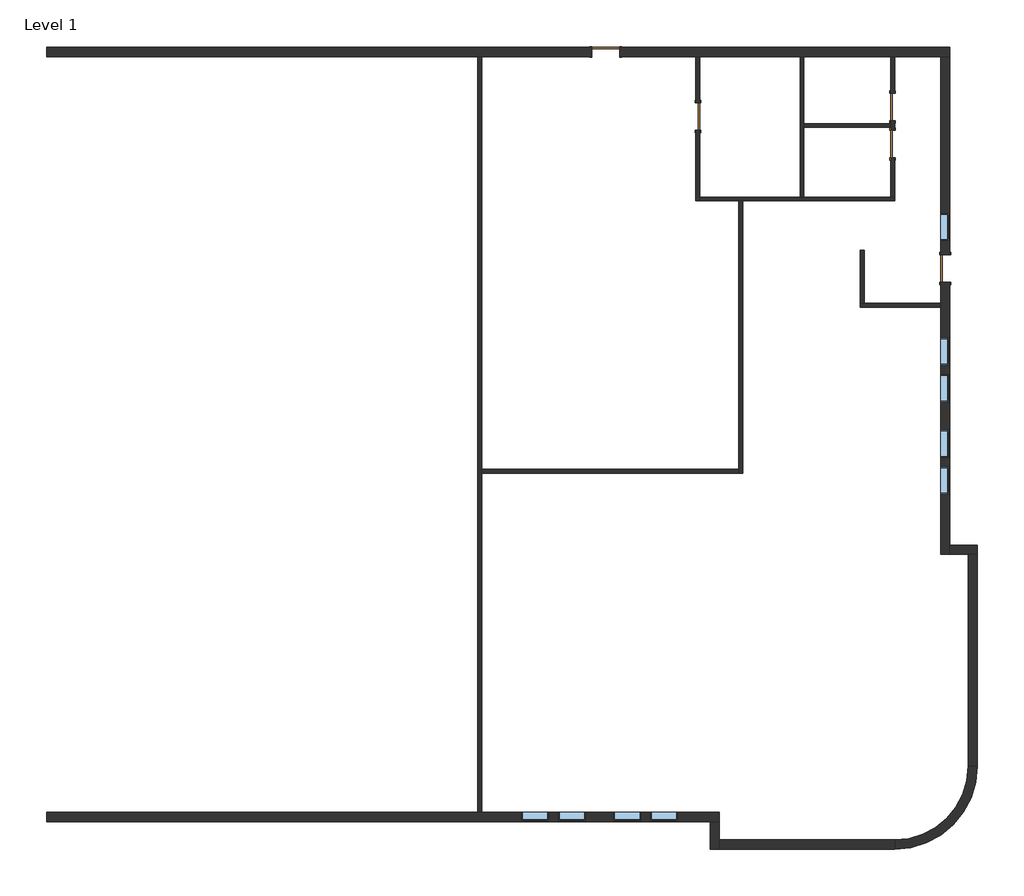
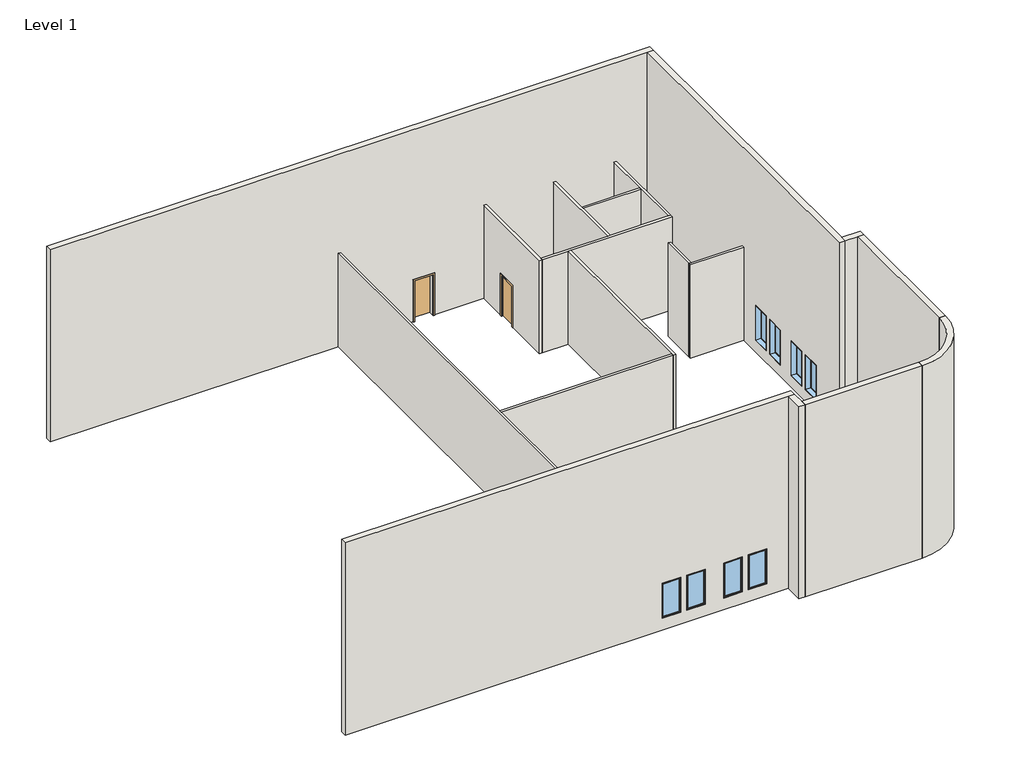
# One storey: 18 walls, 9 windows, 5 doors.
"""IFC4 building model written with IfcOpenShell, lengths in millimetres."""

import ifcopenshell
import ifcopenshell.guid

model = None  # the IFC model being written
_history = None  # IfcOwnerHistory: only IFC2X3 demands one
_inside = {}  # id of a spatial element -> (the spatial element, [elements in it])
_under = {}  # id of a project, library or spatial element -> (it, [spatial elements below it])
_declared = {}  # id of a project -> (the project, [libraries it declares])
_typed = {}  # id of a type object -> (the type object, [elements of that type])
_made_of = {}  # id of a material, layer set ... -> (it, [elements and type objects made of it])


def new_model(schema):
    """Start an empty IFC model of exactly this schema.

    Asked for "IFC4X3", IfcOpenShell would pick the latest addendum, in which some entities
    have other attributes; the version numbers below select the first issue.
    IFC2X3 requires an IfcOwnerHistory on every rooted entity: one is made here for all.
    """
    global model, _history
    if schema == "IFC4X3":
        model = ifcopenshell.file(schema_version=(4, 3, 0, 0))
    else:
        model = ifcopenshell.file(schema=schema)
    _inside.clear()
    _under.clear()
    _declared.clear()
    _typed.clear()
    _made_of.clear()
    _history = None
    if model.schema == "IFC2X3":
        org = make("IfcOrganization", Name="unknown")
        user = make(
            "IfcPersonAndOrganization",
            ThePerson=make("IfcPerson", FamilyName="unknown"),
            TheOrganization=org,
        )
        app = make(
            "IfcApplication",
            ApplicationDeveloper=org,
            Version="unknown",
            ApplicationFullName="unknown",
            ApplicationIdentifier="unknown",
        )
        _history = make(
            "IfcOwnerHistory",
            OwningUser=user,
            OwningApplication=app,
            ChangeAction="ADDED",
            CreationDate=0,
        )
    return model


def make(cls, **values):
    """One entity of the class cls with the attributes given. An attribute that is None is left unset."""
    return model.create_entity(
        cls, **{name: value for name, value in values.items() if value is not None}
    )


def rooted(cls, **values):
    """An entity with a GlobalId (a new one), such as an element, a storey or a relation."""
    return make(cls, GlobalId=ifcopenshell.guid.new(), OwnerHistory=_history, **values)


def si_unit(unit_type, name, prefix=None):
    """IfcSIUnit, for example si_unit("LENGTHUNIT", "METRE", prefix="MILLI")."""
    return make("IfcSIUnit", UnitType=unit_type, Prefix=prefix, Name=name)


def assignment(units):
    """IfcUnitAssignment: the units of a project."""
    return None if units is None else make("IfcUnitAssignment", Units=units)


def point(xyz):
    """IfcCartesianPoint."""
    return None if xyz is None else make("IfcCartesianPoint", Coordinates=xyz)


def direction(xyz):
    """IfcDirection."""
    return None if xyz is None else make("IfcDirection", DirectionRatios=xyz)


def frame(location, z_axis=None, x_axis=None):
    """IfcAxis2Placement3D, a coordinate frame: its origin and axes. An axis left out is left unset."""
    return make(
        "IfcAxis2Placement3D",
        Location=point(location),
        Axis=direction(z_axis),
        RefDirection=direction(x_axis),
    )


def frame_2d(location, x_axis=None):
    """IfcAxis2Placement2D, a coordinate frame in the plane: its origin and x axis."""
    return make(
        "IfcAxis2Placement2D", Location=point(location), RefDirection=direction(x_axis)
    )


def origin():
    """The frame at (0, 0, 0) with its axes left unset."""
    return frame((0.0, 0.0, 0.0))


def origin_with_axes():
    """The frame at (0, 0, 0) with the z axis (0, 0, 1) and the x axis (1, 0, 0) written out."""
    return frame((0.0, 0.0, 0.0), z_axis=(0.0, 0.0, 1.0), x_axis=(1.0, 0.0, 0.0))


def place(relative_to, where):
    """IfcLocalPlacement: puts the frame where relative to a parent placement (None: the world)."""
    return make(
        "IfcLocalPlacement", PlacementRelTo=relative_to, RelativePlacement=where
    )


def context(
    kind, dimensions, precision=None, world=None, true_north=None, identifier=None
):
    """IfcGeometricRepresentationContext, for example the 3D "Model" context."""
    return make(
        "IfcGeometricRepresentationContext",
        ContextIdentifier=identifier,
        ContextType=kind,
        CoordinateSpaceDimension=dimensions,
        Precision=precision,
        WorldCoordinateSystem=world,
        TrueNorth=true_north,
    )


def project(units=None, contexts=None):
    """IfcProject with its units and contexts."""
    return rooted(
        "IfcProject",
        Name="project",
        RepresentationContexts=contexts,
        UnitsInContext=assignment(units),
    )


def spatial(cls, under=None, at=None, **own):
    """A site, building, storey or space (cls), placed at a placement, below another one or the project."""
    s = rooted(cls, ObjectPlacement=at, **own)
    if under is not None:
        _under.setdefault(under.id(), (under, []))[1].append(s)
    return s


def polyline(points):
    """IfcPolyline through the points."""
    return make("IfcPolyline", Points=[point(p) for p in points])


def circle_curve(where, radius):
    """IfcCircle in the frame where."""
    return make("IfcCircle", Position=where, Radius=radius)


def trimmed(basis, trim1, trim2, sense, master):
    """IfcTrimmedCurve: the piece of a basis curve between two trims."""
    return make(
        "IfcTrimmedCurve",
        BasisCurve=basis,
        Trim1=trim1,
        Trim2=trim2,
        SenseAgreement=sense,
        MasterRepresentation=master,
    )


def segment(curve, same_sense, transition):
    """IfcCompositeCurveSegment."""
    return make(
        "IfcCompositeCurveSegment",
        Transition=transition,
        SameSense=same_sense,
        ParentCurve=curve,
    )


def composite_curve(segments, self_intersect=None):
    """IfcCompositeCurve: segments joined end to end."""
    return make("IfcCompositeCurve", Segments=segments, SelfIntersect=self_intersect)


def outline(outer, holes=None, kind="AREA"):
    """IfcArbitraryClosedProfileDef: a profile drawn as a closed curve; with holes, ...WithVoids."""
    if holes is None:
        return make("IfcArbitraryClosedProfileDef", ProfileType=kind, OuterCurve=outer)
    return make(
        "IfcArbitraryProfileDefWithVoids",
        ProfileType=kind,
        OuterCurve=outer,
        InnerCurves=holes,
    )


def extrude(swept, where, along, depth):
    """IfcExtrudedAreaSolid: the profile swept, set in the frame where, extruded along a direction by depth."""
    return make(
        "IfcExtrudedAreaSolid",
        SweptArea=swept,
        Position=where,
        ExtrudedDirection=direction(along),
        Depth=depth,
    )


def faces_of(points, faces, orient=None, outer=None):
    """IfcFace entities. A face is a list of loops; a loop is a list of indices into points, from 0.

    orient and outer hold one flag for each loop. By default every Orientation is true, the
    first loop of a face is its IfcFaceOuterBound and the others are IfcFaceBound.
    """
    made = []
    for i, loops in enumerate(faces):
        bounds = []
        for j, loop in enumerate(loops):
            is_outer = j == 0 if outer is None else outer[i][j]
            bounds.append(
                make(
                    "IfcFaceOuterBound" if is_outer else "IfcFaceBound",
                    Bound=make("IfcPolyLoop", Polygon=[points[k] for k in loop]),
                    Orientation=True if orient is None else orient[i][j],
                )
            )
        made.append(make("IfcFace", Bounds=bounds))
    return made


def faceted_brep(points, faces, orient=None, outer=None, voids=None):
    """IfcFacetedBrep: a solid bounded by flat faces; with voids (closed shells), ...WithVoids."""
    shared = [point(p) for p in points]
    hull = make("IfcClosedShell", CfsFaces=faces_of(shared, faces, orient, outer))
    if voids is None:
        return make("IfcFacetedBrep", Outer=hull)
    return make(
        "IfcFacetedBrepWithVoids",
        Outer=hull,
        Voids=[
            make(cls, CfsFaces=faces_of(shared, fs, o, b)) for cls, fs, o, b in voids
        ],
    )


def shape(context_of_items, identifier, shape_type, items):
    """IfcShapeRepresentation: the items that make up one representation, for example the "Body"."""
    return make(
        "IfcShapeRepresentation",
        ContextOfItems=context_of_items,
        RepresentationIdentifier=identifier,
        RepresentationType=shape_type,
        Items=items,
    )


def source(mapping_origin, context_of_items, identifier, shape_type, items):
    """IfcRepresentationMap: a shape defined once, which mapped items show again and again."""
    return make(
        "IfcRepresentationMap",
        MappingOrigin=mapping_origin,
        MappedRepresentation=shape(context_of_items, identifier, shape_type, items),
    )


def transform(
    local_origin,
    x_axis=None,
    y_axis=None,
    z_axis=None,
    scale=None,
    scale2=None,
    scale3=None,
    uniform=True,
):
    """IfcCartesianTransformationOperator3D, or its non-uniform kind. x_axis, y_axis, z_axis: its Axis1, 2, 3."""
    if uniform:
        return make(
            "IfcCartesianTransformationOperator3D",
            Axis1=direction(x_axis),
            Axis2=direction(y_axis),
            LocalOrigin=point(local_origin),
            Scale=scale,
            Axis3=direction(z_axis),
        )
    return make(
        "IfcCartesianTransformationOperator3DnonUniform",
        Axis1=direction(x_axis),
        Axis2=direction(y_axis),
        LocalOrigin=point(local_origin),
        Scale=scale,
        Axis3=direction(z_axis),
        Scale2=scale2,
        Scale3=scale3,
    )


def mapped(mapping_source, mapping_target):
    """IfcMappedItem: shows the shape of a source again, moved by a transform."""
    return make(
        "IfcMappedItem", MappingSource=mapping_source, MappingTarget=mapping_target
    )


def made_of(thing, what):
    """Note that an element or type object is made of a material, layer set ...; save() writes the relation."""
    if what is not None:
        _made_of.setdefault(what.id(), (what, []))[1].append(thing)
    return thing


def element(
    cls,
    number,
    at=None,
    inside=None,
    cuts=None,
    type_object=None,
    material=None,
    context=None,
    identifier="Body",
    shape_type=None,
    held_by="IfcProductDefinitionShape",
    body=None,
    shapes=None,
    **own,
):
    """One element of the class cls, such as IfcWall. Its Tag is "e" and its number.

    at: its placement. inside: the storey or other place that contains it. cuts: it is an
    opening in that element (IfcRelVoidsElement). A single representation is given by context,
    identifier, shape_type and body (its items); several are given by shapes. held_by: the class
    of the entity that holds the representations. save() writes the other relations.
    """
    e = rooted(cls, Tag="e%d" % number, ObjectPlacement=at, **own)
    if body is not None:
        shapes = [shape(context, identifier, shape_type, body)]
    if shapes is not None:
        e.Representation = make(held_by, Representations=shapes)
    if inside is not None:
        _inside.setdefault(inside.id(), (inside, []))[1].append(e)
    if cuts is not None:
        rooted(
            "IfcRelVoidsElement", RelatingBuildingElement=cuts, RelatedOpeningElement=e
        )
    if type_object is not None:
        _typed.setdefault(type_object.id(), (type_object, []))[1].append(e)
    return made_of(e, material)


def aggregate(whole, parts):
    """IfcRelAggregates: a whole, such as a stair, and the parts it consists of."""
    return rooted("IfcRelAggregates", RelatingObject=whole, RelatedObjects=parts)


def save(model, path):
    """Write the relations noted so far, then the file.

    IfcRelAggregates (storeys below a building ...), IfcRelContainedInSpatialStructure (elements
    in a storey), IfcRelDefinesByType, IfcRelAssociatesMaterial and IfcRelDeclares: one each for
    every whole, place, type object, material and project.
    """
    for whole, parts in _under.values():
        aggregate(whole, parts)
    for where, things in _inside.values():
        rooted(
            "IfcRelContainedInSpatialStructure",
            RelatedElements=things,
            RelatingStructure=where,
        )
    for kind, things in _typed.values():
        rooted("IfcRelDefinesByType", RelatedObjects=things, RelatingType=kind)
    for what, things in _made_of.values():
        rooted("IfcRelAssociatesMaterial", RelatedObjects=things, RelatingMaterial=what)
    for by, libraries in _declared.values():
        rooted("IfcRelDeclares", RelatingContext=by, RelatedDefinitions=libraries)
    model.write(path)


def door_2bf94977(model_context):
    return source(origin(), model_context, "Body", "SweptSolid", [
        extrude(outline(polyline([(2209.8, -533.4), (0.0, -533.4), (0.0, -457.2), (2133.6, -457.2), (2133.6, 457.2), (0.0, 457.2), (0.0, 533.4), (2209.8, 533.4), (2209.8, -533.4)])), frame((0.0, -177.8, 0.0), z_axis=(0.0, 1.0, 0.0), x_axis=(0.0, 0.0, 1.0)), (0.0, 0.0, 1.0), 25.4),
        extrude(outline(polyline([(2209.8, 533.4), (2209.8, -533.4), (0.0, -533.4), (0.0, -457.2), (2133.6, -457.2), (2133.6, 457.2), (0.0, 457.2), (0.0, 533.4), (2209.8, 533.4)])), frame((0.0, 152.4, 0.0), z_axis=(0.0, 1.0, 0.0), x_axis=(0.0, 0.0, 1.0)), (0.0, 0.0, 1.0), 25.4),
        extrude(outline(polyline([(457.2, -101.6), (457.2, -152.4), (-457.2, -152.4), (-457.2, -101.6), (457.2, -101.6)])), origin_with_axes(), (0.0, 0.0, 1.0), 2133.6),
    ])


def door_a3eb833a(model_context):
    return source(origin(), model_context, "Body", "SweptSolid", [
        extrude(outline(polyline([(2209.8, -533.4), (0.0, -533.4), (0.0, -457.2), (2133.6, -457.2), (2133.6, 457.2), (0.0, 457.2), (0.0, 533.4), (2209.8, 533.4), (2209.8, -533.4)])), frame((0.0, -88.9, 0.0), z_axis=(0.0, 1.0, 0.0), x_axis=(0.0, 0.0, 1.0)), (0.0, 0.0, 1.0), 25.4),
        extrude(outline(polyline([(2209.8, 533.4), (2209.8, -533.4), (0.0, -533.4), (0.0, -457.2), (2133.6, -457.2), (2133.6, 457.2), (0.0, 457.2), (0.0, 533.4), (2209.8, 533.4)])), frame((0.0, 63.5, 0.0), z_axis=(0.0, 1.0, 0.0), x_axis=(0.0, 0.0, 1.0)), (0.0, 0.0, 1.0), 25.4),
        extrude(outline(polyline([(457.2, -12.7), (457.2, -63.5), (-457.2, -63.5), (-457.2, -12.7), (457.2, -12.7)])), origin_with_axes(), (0.0, 0.0, 1.0), 2133.6),
    ])


def door_a1797ceb(model_context):
    return source(origin(), model_context, "Body", "SweptSolid", [
        extrude(outline(polyline([(2209.8, -533.4), (0.0, -533.4), (0.0, -457.2), (2133.6, -457.2), (2133.6, 457.2), (0.0, 457.2), (0.0, 533.4), (2209.8, 533.4), (2209.8, -533.4)])), frame((0.0, 63.5, 0.0), z_axis=(0.0, 1.0, 0.0), x_axis=(0.0, 0.0, 1.0)), (0.0, 0.0, 1.0), 25.4),
        extrude(outline(polyline([(2209.8, 533.4), (2209.8, -533.4), (0.0, -533.4), (0.0, -457.2), (2133.6, -457.2), (2133.6, 457.2), (0.0, 457.2), (0.0, 533.4), (2209.8, 533.4)])), frame((0.0, -88.9, 0.0), z_axis=(0.0, 1.0, 0.0), x_axis=(0.0, 0.0, 1.0)), (0.0, 0.0, 1.0), 25.4),
        extrude(outline(polyline([(457.2, 12.7), (-457.2, 12.7), (-457.2, 63.5), (457.2, 63.5), (457.2, 12.7)])), origin_with_axes(), (0.0, 0.0, 1.0), 2133.6),
    ])


def window_c524ad49(model_context):
    return source(origin(), model_context, "Body", "SweptSolid", [
        extrude(outline(polyline([(355.6, 104.775), (-431.8, 104.775), (-431.8, 117.475), (355.6, 117.475), (355.6, 104.775)])), frame((0.0, 0.0, 368.3), z_axis=(0.0, 0.0, 1.0), x_axis=(1.0, 0.0, 0.0)), (0.0, 0.0, 1.0), 1701.8),
        extrude(outline(polyline([(2114.55, -476.25), (323.85, -476.25), (323.85, 400.05), (2114.55, 400.05), (2114.55, -476.25)]), holes=[polyline([(2070.1, -431.8), (2070.1, 355.6), (368.3, 355.6), (368.3, -431.8), (2070.1, -431.8)])]), frame((0.0, 88.9, 0.0), z_axis=(0.0, 1.0, 0.0), x_axis=(0.0, 0.0, 1.0)), (0.0, 0.0, 1.0), 44.45),
        extrude(outline(polyline([(2133.6, -495.3), (304.8, -495.3), (304.8, 419.1), (2133.6, 419.1), (2133.6, -495.3)]), holes=[polyline([(2101.85, -463.55), (2101.85, 387.35), (336.55, 387.35), (336.55, -463.55), (2101.85, -463.55)])]), frame((0.0, -152.4, 0.0), z_axis=(0.0, 1.0, 0.0), x_axis=(0.0, 0.0, 1.0)), (0.0, 0.0, 1.0), 241.3),
        extrude(outline(polyline([(2133.6, 419.1), (2133.6, -495.3), (304.8, -495.3), (304.8, 419.1), (2133.6, 419.1)]), holes=[polyline([(2114.55, 400.05), (323.85, 400.05), (323.85, -476.25), (2114.55, -476.25), (2114.55, 400.05)])]), frame((0.0, 88.9, 0.0), z_axis=(0.0, 1.0, 0.0), x_axis=(0.0, 0.0, 1.0)), (0.0, 0.0, 1.0), 63.5),
    ])


def window_9a1f8bc2(model_context):
    return source(origin(), model_context, "Body", "SweptSolid", [
        extrude(outline(polyline([(355.6, -104.775), (355.6, -117.475), (-431.8, -117.475), (-431.8, -104.775), (355.6, -104.775)])), frame((0.0, 0.0, 368.3), z_axis=(0.0, 0.0, 1.0), x_axis=(1.0, 0.0, 0.0)), (0.0, 0.0, 1.0), 1701.8),
        extrude(outline(polyline([(2114.55, -476.25), (323.85, -476.25), (323.85, 400.05), (2114.55, 400.05), (2114.55, -476.25)]), holes=[polyline([(2070.1, -431.8), (2070.1, 355.6), (368.3, 355.6), (368.3, -431.8), (2070.1, -431.8)])]), frame((0.0, -133.35, 0.0), z_axis=(0.0, 1.0, 0.0), x_axis=(0.0, 0.0, 1.0)), (0.0, 0.0, 1.0), 44.45),
        extrude(outline(polyline([(2133.6, -495.3), (304.8, -495.3), (304.8, 419.1), (2133.6, 419.1), (2133.6, -495.3)]), holes=[polyline([(2101.85, -463.55), (2101.85, 387.35), (336.55, 387.35), (336.55, -463.55), (2101.85, -463.55)])]), frame((0.0, -88.9, 0.0), z_axis=(0.0, 1.0, 0.0), x_axis=(0.0, 0.0, 1.0)), (0.0, 0.0, 1.0), 241.3),
        extrude(outline(polyline([(2133.6, 419.1), (2133.6, -495.3), (304.8, -495.3), (304.8, 419.1), (2133.6, 419.1)]), holes=[polyline([(2114.55, 400.05), (323.85, 400.05), (323.85, -476.25), (2114.55, -476.25), (2114.55, 400.05)])]), frame((0.0, -152.4, 0.0), z_axis=(0.0, 1.0, 0.0), x_axis=(0.0, 0.0, 1.0)), (0.0, 0.0, 1.0), 63.5),
    ])


model = new_model("IFC4")

# Units and contexts
model_context = context("Model", 3, world=origin())
ifc_project = project(units=[si_unit("LENGTHUNIT", "METRE", prefix="MILLI")], contexts=[model_context])

# Site, building, storey
site = spatial("IfcSite", under=ifc_project)
building = spatial("IfcBuilding", under=site)
storey = spatial("IfcBuildingStorey", under=building, Name="Level 1", Elevation=0.0)

# Doors
placement = place(None, origin())
door_shape = door_2bf94977(model_context)
element("IfcDoor", 1, ObjectType="Single-Flush : 36\" x 84\"", at=placement, inside=storey, context=model_context, shape_type="MappedRepresentation", body=[
    mapped(door_shape, transform((7004.4737178, 13634.9120281, 0.0), x_axis=(-1.0, 0.0, 0.0), y_axis=(0.0, -1.0, 0.0), z_axis=(0.0, 0.0, 1.0))),
])
element("IfcDoor", 2, ObjectType="Single-Flush : 36\" x 84\"", at=placement, inside=storey, context=model_context, shape_type="MappedRepresentation", body=[
    mapped(door_shape, transform((18231.2737178, 6472.1120281, 0.0), x_axis=(0.0, -1.0, 0.0), y_axis=(1.0, 0.0, 0.0), z_axis=(0.0, 0.0, 1.0))),
])
door_2_shape = door_a3eb833a(model_context)
element("IfcDoor", 3, ObjectType="Single-Flush : 36\" x 84\"", at=placement, inside=storey, context=model_context, shape_type="MappedRepresentation", body=[
    mapped(door_2_shape, transform((16491.3737178, 11812.4620281, 0.0), x_axis=(0.0, -1.0, 0.0), y_axis=(1.0, 0.0, 0.0), z_axis=(0.0, 0.0, 1.0))),
])
element("IfcDoor", 4, ObjectType="Single-Flush : 36\" x 84\"", at=placement, inside=storey, context=model_context, shape_type="MappedRepresentation", body=[
    mapped(door_2_shape, transform((10052.4737178, 11501.3120281, 0.0), x_axis=(0.0, 1.0, 0.0), y_axis=(-1.0, 0.0, 0.0), z_axis=(0.0, 0.0, 1.0))),
])
door_3_shape = door_a1797ceb(model_context)
element("IfcDoor", 5, ObjectType="Single-Flush : 36\" x 84\"", at=placement, inside=storey, context=model_context, shape_type="MappedRepresentation", body=[
    mapped(door_3_shape, transform((16491.3737178, 10593.2620281, 0.0), x_axis=(0.0, 1.0, 0.0), y_axis=(-1.0, 0.0, 0.0), z_axis=(0.0, 0.0, 1.0))),
])

# Walls
element("IfcWall", 6, ObjectType="Generic - 12\"", at=placement, inside=storey, context=model_context, shape_type="Brep", body=[
    faceted_brep([(-11486.7262822, 13482.5120281, 0.0), (2775.3737178, 13482.5120281, 0.0), (2902.3737178, 13482.5120281, 0.0), (6547.2737178, 13482.5120281, 0.0), (6547.2737178, 13482.5120281, 2133.6), (7461.6737178, 13482.5120281, 2133.6), (7461.6737178, 13482.5120281, 0.0), (9988.9737178, 13482.5120281, 0.0), (10115.9737178, 13482.5120281, 0.0), (13430.6737178, 13482.5120281, 0.0), (13557.6737178, 13482.5120281, 0.0), (16427.8737178, 13482.5120281, 0.0), (16554.8737178, 13482.5120281, 0.0), (18078.8737178, 13482.5120281, 0.0), (18383.6737178, 13482.5120281, 0.0), (18383.6737178, 13482.5120281, 10058.4), (18078.8737178, 13482.5120281, 10058.4), (-11486.7262822, 13482.5120281, 10058.4), (6547.2737178, 13787.3120281, 2133.6), (6547.2737178, 13787.3120281, 0.0), (-11486.7262822, 13787.3120281, 0.0), (-11486.7262822, 13787.3120281, 10058.4), (18383.6737178, 13787.3120281, 10058.4), (18383.6737178, 13787.3120281, 0.0), (7461.6737178, 13787.3120281, 0.0), (7461.6737178, 13787.3120281, 2133.6)], [[[0, 1, 2, 3, 4, 5, 6, 7, 8, 9, 10, 11, 12, 13, 14, 15, 16, 17]], [[18, 19, 20, 21, 22, 23, 24, 25]], [[24, 23, 14, 13, 12, 11, 10, 9, 8, 7, 6]], [[20, 19, 3, 2, 1, 0]], [[17, 16, 15, 22, 21]], [[0, 17, 21, 20]], [[15, 14, 23, 22]], [[4, 3, 19, 18]], [[5, 4, 18, 25]], [[6, 5, 25, 24]]]),
])
element("IfcWall", 7, ObjectType="Generic - 12\"", at=placement, inside=storey, context=model_context, shape_type="Brep", body=[
    faceted_brep([(18078.8737178, 6014.9120281, 2133.6), (18078.8737178, 6014.9120281, 0.0), (18078.8737178, 5316.4120281, 0.0), (18078.8737178, 5189.4120281, 0.0), (18078.8737178, -2976.6879719, 0.0), (18078.8737178, -2976.6879719, 10058.4), (18078.8737178, 13482.5120281, 10058.4), (18078.8737178, 13482.5120281, 0.0), (18078.8737178, 6929.3120281, 0.0), (18078.8737178, 6929.3120281, 2133.6), (18078.8737178, -995.4879719, 2438.4), (18078.8737178, -995.4879719, 609.6), (18078.8737178, -81.0879719, 609.6), (18078.8737178, -81.0879719, 2438.4), (18078.8737178, 223.7120281, 2438.4), (18078.8737178, 223.7120281, 609.6), (18078.8737178, 1138.1120281, 609.6), (18078.8737178, 1138.1120281, 2438.4), (18078.8737178, 2052.5120281, 2438.4), (18078.8737178, 2052.5120281, 609.6), (18078.8737178, 2966.9120281, 609.6), (18078.8737178, 2966.9120281, 2438.4), (18078.8737178, 3271.7120281, 2438.4), (18078.8737178, 3271.7120281, 609.6), (18078.8737178, 4186.1120281, 609.6), (18078.8737178, 4186.1120281, 2438.4), (18078.8737178, 7386.5120281, 2438.4), (18078.8737178, 7386.5120281, 609.6), (18078.8737178, 8300.9120281, 609.6), (18078.8737178, 8300.9120281, 2438.4), (18383.6737178, -2976.6879719, 0.0), (18383.6737178, -2671.8879719, 0.0), (18383.6737178, 6014.9120281, 0.0), (18383.6737178, 6014.9120281, 2133.6), (18383.6737178, 6929.3120281, 2133.6), (18383.6737178, 6929.3120281, 0.0), (18383.6737178, 13482.5120281, 0.0), (18383.6737178, 13482.5120281, 10058.4), (18383.6737178, -2671.8879719, 10058.4), (18383.6737178, -2976.6879719, 10058.4), (18383.6737178, -995.4879719, 2438.4), (18383.6737178, -81.0879719, 2438.4), (18383.6737178, -81.0879719, 609.6), (18383.6737178, -995.4879719, 609.6), (18383.6737178, 223.7120281, 2438.4), (18383.6737178, 1138.1120281, 2438.4), (18383.6737178, 1138.1120281, 609.6), (18383.6737178, 223.7120281, 609.6), (18383.6737178, 2052.5120281, 2438.4), (18383.6737178, 2966.9120281, 2438.4), (18383.6737178, 2966.9120281, 609.6), (18383.6737178, 2052.5120281, 609.6), (18383.6737178, 3271.7120281, 2438.4), (18383.6737178, 4186.1120281, 2438.4), (18383.6737178, 4186.1120281, 609.6), (18383.6737178, 3271.7120281, 609.6), (18383.6737178, 7386.5120281, 2438.4), (18383.6737178, 8300.9120281, 2438.4), (18383.6737178, 8300.9120281, 609.6), (18383.6737178, 7386.5120281, 609.6)], [[[0, 1, 2, 3, 4, 5, 6, 7, 8, 9], [10, 11, 12, 13], [14, 15, 16, 17], [18, 19, 20, 21], [22, 23, 24, 25], [26, 27, 28, 29]], [[30, 31, 32, 33, 34, 35, 36, 37, 38, 39], [40, 41, 42, 43], [44, 45, 46, 47], [48, 49, 50, 51], [52, 53, 54, 55], [56, 57, 58, 59]], [[8, 7, 36, 35]], [[4, 3, 2, 1, 32, 31, 30]], [[6, 5, 39, 38, 37]], [[7, 6, 37, 36]], [[11, 10, 40, 43]], [[12, 11, 43, 42]], [[13, 12, 42, 41]], [[10, 13, 41, 40]], [[15, 14, 44, 47]], [[16, 15, 47, 46]], [[17, 16, 46, 45]], [[14, 17, 45, 44]], [[19, 18, 48, 51]], [[20, 19, 51, 50]], [[21, 20, 50, 49]], [[18, 21, 49, 48]], [[23, 22, 52, 55]], [[24, 23, 55, 54]], [[25, 24, 54, 53]], [[22, 25, 53, 52]], [[27, 26, 56, 59]], [[28, 27, 59, 58]], [[29, 28, 58, 57]], [[26, 29, 57, 56]], [[33, 32, 1, 0]], [[34, 33, 0, 9]], [[35, 34, 9, 8]], [[5, 4, 30, 39]]]),
])
element("IfcWall", 8, ObjectType="Generic - 12\"", at=placement, inside=storey, context=model_context, shape_type="Brep", body=[
    faceted_brep([(10763.6737178, -11511.0879719, 0.0), (2902.3737178, -11511.0879719, 0.0), (2775.3737178, -11511.0879719, 0.0), (-11486.7262822, -11511.0879719, 0.0), (-11486.7262822, -11511.0879719, 10058.4), (10763.6737178, -11511.0879719, 10058.4), (9392.0737178, -11511.0879719, 2438.4), (8477.6737178, -11511.0879719, 2438.4), (8477.6737178, -11511.0879719, 609.6), (9392.0737178, -11511.0879719, 609.6), (8172.8737178, -11511.0879719, 2438.4), (7258.4737178, -11511.0879719, 2438.4), (7258.4737178, -11511.0879719, 609.6), (8172.8737178, -11511.0879719, 609.6), (6344.0737178, -11511.0879719, 2438.4), (5429.6737178, -11511.0879719, 2438.4), (5429.6737178, -11511.0879719, 609.6), (6344.0737178, -11511.0879719, 609.6), (5124.8737178, -11511.0879719, 2438.4), (4210.4737178, -11511.0879719, 2438.4), (4210.4737178, -11511.0879719, 609.6), (5124.8737178, -11511.0879719, 609.6), (10763.6737178, -11815.8879719, 0.0), (10763.6737178, -11815.8879719, 10058.4), (10458.8737178, -11815.8879719, 10058.4), (-11486.7262822, -11815.8879719, 10058.4), (-11486.7262822, -11815.8879719, 0.0), (10458.8737178, -11815.8879719, 0.0), (9392.0737178, -11815.8879719, 2438.4), (9392.0737178, -11815.8879719, 609.6), (8477.6737178, -11815.8879719, 609.6), (8477.6737178, -11815.8879719, 2438.4), (8172.8737178, -11815.8879719, 2438.4), (8172.8737178, -11815.8879719, 609.6), (7258.4737178, -11815.8879719, 609.6), (7258.4737178, -11815.8879719, 2438.4), (6344.0737178, -11815.8879719, 2438.4), (6344.0737178, -11815.8879719, 609.6), (5429.6737178, -11815.8879719, 609.6), (5429.6737178, -11815.8879719, 2438.4), (5124.8737178, -11815.8879719, 2438.4), (5124.8737178, -11815.8879719, 609.6), (4210.4737178, -11815.8879719, 609.6), (4210.4737178, -11815.8879719, 2438.4)], [[[0, 1, 2, 3, 4, 5], [6, 7, 8, 9], [10, 11, 12, 13], [14, 15, 16, 17], [18, 19, 20, 21]], [[22, 23, 24, 25, 26, 27], [28, 29, 30, 31], [32, 33, 34, 35], [36, 37, 38, 39], [40, 41, 42, 43]], [[3, 2, 1, 0, 22, 27, 26]], [[4, 3, 26, 25]], [[5, 4, 25, 24, 23]], [[29, 28, 6, 9]], [[30, 29, 9, 8]], [[31, 30, 8, 7]], [[28, 31, 7, 6]], [[33, 32, 10, 13]], [[34, 33, 13, 12]], [[35, 34, 12, 11]], [[32, 35, 11, 10]], [[37, 36, 14, 17]], [[38, 37, 17, 16]], [[39, 38, 16, 15]], [[36, 39, 15, 14]], [[41, 40, 18, 21]], [[42, 41, 21, 20]], [[43, 42, 20, 19]], [[40, 43, 19, 18]], [[0, 5, 23, 22]]]),
])
element("IfcWall", 9, ObjectType="Generic - 12\"", at=placement, inside=storey, context=model_context, shape_type="Brep", body=[
    faceted_brep([(10458.8737178, -11815.8879719, 0.0), (10458.8737178, -12730.2879719, 0.0), (10458.8737178, -12730.2879719, 10058.4), (10458.8737178, -11815.8879719, 10058.4), (10763.6737178, -11815.8879719, 0.0), (10763.6737178, -11815.8879719, 10058.4), (10763.6737178, -12425.4879719, 10058.4), (10763.6737178, -12730.2879719, 10058.4), (10763.6737178, -12730.2879719, 0.0), (10763.6737178, -12425.4879719, 0.0)], [[[0, 1, 2, 3]], [[4, 5, 6, 7, 8, 9]], [[1, 0, 4, 9, 8]], [[3, 2, 7, 6, 5]], [[2, 1, 8, 7]], [[0, 3, 5, 4]]]),
])
element("IfcWall", 10, ObjectType="Generic - 12\"", at=placement, inside=storey, context=model_context, shape_type="SweptSolid", body=[
    extrude(outline(polyline([(16554.8737178, -12730.2879719), (10763.6737178, -12730.2879719), (10763.6737178, -12425.4879719), (16554.8737178, -12425.4879719), (16554.8737178, -12730.2879719)])), origin_with_axes(), (0.0, 0.0, 1.0), 10058.4),
])
element("IfcWall", 11, ObjectType="Generic - 12\"", at=placement, inside=storey, context=model_context, shape_type="Brep", body=[
    faceted_brep([(18383.6737178, -2976.6879719, 0.0), (18993.2737178, -2976.6879719, 0.0), (19298.0737178, -2976.6879719, 0.0), (19298.0737178, -2976.6879719, 10058.4), (18993.2737178, -2976.6879719, 10058.4), (18383.6737178, -2976.6879719, 10058.4), (18383.6737178, -2671.8879719, 0.0), (18383.6737178, -2671.8879719, 10058.4), (19298.0737178, -2671.8879719, 10058.4), (19298.0737178, -2671.8879719, 0.0)], [[[0, 1, 2, 3, 4, 5]], [[6, 7, 8, 9]], [[2, 1, 0, 6, 9]], [[5, 4, 3, 8, 7]], [[3, 2, 9, 8]], [[0, 5, 7, 6]]]),
])
element("IfcWall", 12, ObjectType="Generic - 12\"", at=placement, inside=storey, context=model_context, shape_type="SweptSolid", body=[
    extrude(outline(polyline([(18993.2737178, -9987.0879719), (18993.2737178, -2976.6879719), (19298.0737178, -2976.6879719), (19298.0737178, -9987.0879719), (18993.2737178, -9987.0879719)])), origin_with_axes(), (0.0, 0.0, 1.0), 10058.4),
])
element("IfcWall", 13, ObjectType="Generic - 12\"", at=placement, inside=storey, context=model_context, shape_type="SweptSolid", body=[
    extrude(outline(composite_curve([segment(polyline([(18993.2737178, -9987.0879719), (19298.0737178, -9987.0879719)]), True, "CONTINUOUS"), segment(trimmed(circle_curve(frame_2d((16554.8737178, -9987.0879719)), 2743.2), [point((19298.0737178, -9987.0879719))], [point((16554.8737178, -12730.2879719))], False, "CARTESIAN"), True, "CONTINUOUS"), segment(polyline([(16554.8737178, -12730.2879719), (16554.8737178, -12425.4879719)]), True, "CONTINUOUS"), segment(trimmed(circle_curve(frame_2d((16554.8737178, -9987.0879719)), 2438.4), [point((16554.8737178, -12425.4879719))], [point((18993.2737178, -9987.0879719))], True, "CARTESIAN"), True, "CONTINUOUS")], self_intersect=False)), origin_with_axes(), (0.0, 0.0, 1.0), 10058.4),
])
element("IfcWall", 14, ObjectType="Generic - 5\"", at=placement, inside=storey, context=model_context, shape_type="Brep", body=[
    faceted_brep([(2902.3737178, -11511.0879719, 0.0), (2902.3737178, -296.9879719, 0.0), (2902.3737178, -169.9879719, 0.0), (2902.3737178, 13482.5120281, 0.0), (2902.3737178, 13482.5120281, 4876.8), (2902.3737178, -169.9879719, 4876.8), (2902.3737178, -296.9879719, 4876.8), (2902.3737178, -11511.0879719, 4876.8), (2775.3737178, -11511.0879719, 0.0), (2775.3737178, -11511.0879719, 4876.8), (2775.3737178, 13482.5120281, 4876.8), (2775.3737178, 13482.5120281, 0.0)], [[[0, 1, 2, 3, 4, 5, 6, 7]], [[8, 9, 10, 11]], [[3, 2, 1, 0, 8, 11]], [[7, 6, 5, 4, 10, 9]], [[4, 3, 11, 10]], [[0, 7, 9, 8]]]),
])
element("IfcWall", 15, ObjectType="Generic - 5\"", at=placement, inside=storey, context=model_context, shape_type="Brep", body=[
    faceted_brep([(9988.9737178, 13482.5120281, 0.0), (9988.9737178, 11958.5120281, 0.0), (9988.9737178, 11958.5120281, 2133.6), (9988.9737178, 11044.1120281, 2133.6), (9988.9737178, 11044.1120281, 0.0), (9988.9737178, 8707.3120281, 0.0), (9988.9737178, 8707.3120281, 4876.8), (9988.9737178, 13482.5120281, 4876.8), (10115.9737178, 11958.5120281, 2133.6), (10115.9737178, 11958.5120281, 0.0), (10115.9737178, 13482.5120281, 0.0), (10115.9737178, 13482.5120281, 4876.8), (10115.9737178, 8834.3120281, 4876.8), (10115.9737178, 8707.3120281, 4876.8), (10115.9737178, 8707.3120281, 0.0), (10115.9737178, 8834.3120281, 0.0), (10115.9737178, 11044.1120281, 0.0), (10115.9737178, 11044.1120281, 2133.6)], [[[0, 1, 2, 3, 4, 5, 6, 7]], [[8, 9, 10, 11, 12, 13, 14, 15, 16, 17]], [[10, 9, 1, 0]], [[16, 15, 14, 5, 4]], [[7, 6, 13, 12, 11]], [[0, 7, 11, 10]], [[6, 5, 14, 13]], [[2, 1, 9, 8]], [[3, 2, 8, 17]], [[4, 3, 17, 16]]]),
])
element("IfcWall", 16, ObjectType="Generic - 5\"", at=placement, inside=storey, context=model_context, shape_type="Brep", body=[
    faceted_brep([(10115.9737178, 8707.3120281, 0.0), (11411.3737178, 8707.3120281, 0.0), (11538.3737178, 8707.3120281, 0.0), (16554.8737178, 8707.3120281, 0.0), (16554.8737178, 8707.3120281, 4876.8), (11538.3737178, 8707.3120281, 4876.8), (11411.3737178, 8707.3120281, 4876.8), (10115.9737178, 8707.3120281, 4876.8), (10115.9737178, 8834.3120281, 0.0), (10115.9737178, 8834.3120281, 4876.8), (13430.6737178, 8834.3120281, 4876.8), (13557.6737178, 8834.3120281, 4876.8), (16427.8737178, 8834.3120281, 4876.8), (16554.8737178, 8834.3120281, 4876.8), (16554.8737178, 8834.3120281, 0.0), (16427.8737178, 8834.3120281, 0.0), (13557.6737178, 8834.3120281, 0.0), (13430.6737178, 8834.3120281, 0.0)], [[[0, 1, 2, 3, 4, 5, 6, 7]], [[8, 9, 10, 11, 12, 13, 14, 15, 16, 17]], [[3, 2, 1, 0, 8, 17, 16, 15, 14]], [[7, 6, 5, 4, 13, 12, 11, 10, 9]], [[0, 7, 9, 8]], [[4, 3, 14, 13]]]),
])
element("IfcWall", 17, ObjectType="Generic - 5\"", at=placement, inside=storey, context=model_context, shape_type="Brep", body=[
    faceted_brep([(16554.8737178, 11050.4620281, 2133.6), (16554.8737178, 11050.4620281, 0.0), (16554.8737178, 11355.2620281, 0.0), (16554.8737178, 11355.2620281, 2133.6), (16554.8737178, 12269.6620281, 2133.6), (16554.8737178, 12269.6620281, 0.0), (16554.8737178, 13482.5120281, 0.0), (16554.8737178, 13482.5120281, 4876.8), (16554.8737178, 8834.3120281, 4876.8), (16554.8737178, 8834.3120281, 0.0), (16554.8737178, 10136.0620281, 0.0), (16554.8737178, 10136.0620281, 2133.6), (16427.8737178, 11355.2620281, 0.0), (16427.8737178, 11266.3620281, 0.0), (16427.8737178, 11139.3620281, 0.0), (16427.8737178, 11050.4620281, 0.0), (16427.8737178, 11050.4620281, 2133.6), (16427.8737178, 10136.0620281, 2133.6), (16427.8737178, 10136.0620281, 0.0), (16427.8737178, 8834.3120281, 0.0), (16427.8737178, 8834.3120281, 4876.8), (16427.8737178, 11139.3620281, 4876.8), (16427.8737178, 11266.3620281, 4876.8), (16427.8737178, 13482.5120281, 4876.8), (16427.8737178, 13482.5120281, 0.0), (16427.8737178, 12269.6620281, 0.0), (16427.8737178, 12269.6620281, 2133.6), (16427.8737178, 11355.2620281, 2133.6)], [[[0, 1, 2, 3, 4, 5, 6, 7, 8, 9, 10, 11]], [[12, 13, 14, 15, 16, 17, 18, 19, 20, 21, 22, 23, 24, 25, 26, 27]], [[25, 24, 6, 5]], [[10, 9, 19, 18]], [[2, 1, 15, 14, 13, 12]], [[8, 7, 23, 22, 21, 20]], [[9, 8, 20, 19]], [[7, 6, 24, 23]], [[16, 15, 1, 0]], [[17, 16, 0, 11]], [[18, 17, 11, 10]], [[3, 2, 12, 27]], [[4, 3, 27, 26]], [[5, 4, 26, 25]]]),
])
element("IfcWall", 18, ObjectType="Generic - 5\"", at=placement, inside=storey, context=model_context, shape_type="Brep", body=[
    faceted_brep([(13430.6737178, 13482.5120281, 0.0), (13430.6737178, 8834.3120281, 0.0), (13430.6737178, 8834.3120281, 4876.8), (13430.6737178, 13482.5120281, 4876.8), (13557.6737178, 13482.5120281, 0.0), (13557.6737178, 13482.5120281, 4876.8), (13557.6737178, 11266.3620281, 4876.8), (13557.6737178, 11139.3620281, 4876.8), (13557.6737178, 8834.3120281, 4876.8), (13557.6737178, 8834.3120281, 0.0), (13557.6737178, 11139.3620281, 0.0), (13557.6737178, 11266.3620281, 0.0)], [[[0, 1, 2, 3]], [[4, 5, 6, 7, 8, 9, 10, 11]], [[1, 0, 4, 11, 10, 9]], [[3, 2, 8, 7, 6, 5]], [[0, 3, 5, 4]], [[2, 1, 9, 8]]]),
])
element("IfcWall", 19, ObjectType="Generic - 5\"", at=placement, inside=storey, context=model_context, shape_type="SweptSolid", body=[
    extrude(outline(polyline([(13557.6737178, 11266.3620281), (16427.8737178, 11266.3620281), (16427.8737178, 11139.3620281), (13557.6737178, 11139.3620281), (13557.6737178, 11266.3620281)])), origin_with_axes(), (0.0, 0.0, 1.0), 4876.8),
])
element("IfcWall", 20, ObjectType="Generic - 5\"", at=placement, inside=storey, context=model_context, shape_type="Brep", body=[
    faceted_brep([(18078.8737178, 5316.4120281, 0.0), (15551.5737178, 5316.4120281, 0.0), (15424.5737178, 5316.4120281, 0.0), (15424.5737178, 5316.4120281, 4876.8), (15551.5737178, 5316.4120281, 4876.8), (18078.8737178, 5316.4120281, 4876.8), (18078.8737178, 5189.4120281, 0.0), (18078.8737178, 5189.4120281, 4876.8), (15424.5737178, 5189.4120281, 4876.8), (15424.5737178, 5189.4120281, 0.0)], [[[0, 1, 2, 3, 4, 5]], [[6, 7, 8, 9]], [[2, 1, 0, 6, 9]], [[5, 4, 3, 8, 7]], [[0, 5, 7, 6]], [[3, 2, 9, 8]]]),
])
element("IfcWall", 21, ObjectType="Generic - 5\"", at=placement, inside=storey, context=model_context, shape_type="SweptSolid", body=[
    extrude(outline(polyline([(15551.5737178, 7081.7120281), (15551.5737178, 5316.4120281), (15424.5737178, 5316.4120281), (15424.5737178, 7081.7120281), (15551.5737178, 7081.7120281)])), origin_with_axes(), (0.0, 0.0, 1.0), 4876.8),
])
element("IfcWall", 22, ObjectType="Generic - 5\"", at=placement, inside=storey, context=model_context, shape_type="Brep", body=[
    faceted_brep([(11411.3737178, 8707.3120281, 0.0), (11411.3737178, -169.9879719, 0.0), (11411.3737178, -296.9879719, 0.0), (11411.3737178, -296.9879719, 4876.8), (11411.3737178, -169.9879719, 4876.8), (11411.3737178, 8707.3120281, 4876.8), (11538.3737178, 8707.3120281, 0.0), (11538.3737178, 8707.3120281, 4876.8), (11538.3737178, -296.9879719, 4876.8), (11538.3737178, -296.9879719, 0.0)], [[[0, 1, 2, 3, 4, 5]], [[6, 7, 8, 9]], [[2, 1, 0, 6, 9]], [[5, 4, 3, 8, 7]], [[0, 5, 7, 6]], [[3, 2, 9, 8]]]),
])
element("IfcWall", 23, ObjectType="Generic - 5\"", at=placement, inside=storey, context=model_context, shape_type="SweptSolid", body=[
    extrude(outline(polyline([(2902.3737178, -169.9879719), (11411.3737178, -169.9879719), (11411.3737178, -296.9879719), (2902.3737178, -296.9879719), (2902.3737178, -169.9879719)])), origin_with_axes(), (0.0, 0.0, 1.0), 4876.8),
])

# Windows
window_shape = window_c524ad49(model_context)
element("IfcWindow", 24, ObjectType="Fixed : 36\" x 72\"", at=placement, inside=storey, context=model_context, shape_type="MappedRepresentation", body=[
    mapped(window_shape, transform((18231.2737178, 7805.6120281, 304.8), x_axis=(0.0, -1.0, 0.0), y_axis=(1.0, 0.0, 0.0), z_axis=(0.0, 0.0, 1.0))),
])
element("IfcWindow", 25, ObjectType="Fixed : 36\" x 72\"", at=placement, inside=storey, context=model_context, shape_type="MappedRepresentation", body=[
    mapped(window_shape, transform((18231.2737178, 3690.8120281, 304.8), x_axis=(0.0, -1.0, 0.0), y_axis=(1.0, 0.0, 0.0), z_axis=(0.0, 0.0, 1.0))),
])
element("IfcWindow", 26, ObjectType="Fixed : 36\" x 72\"", at=placement, inside=storey, context=model_context, shape_type="MappedRepresentation", body=[
    mapped(window_shape, transform((18231.2737178, 2471.6120281, 304.8), x_axis=(0.0, -1.0, 0.0), y_axis=(1.0, 0.0, 0.0), z_axis=(0.0, 0.0, 1.0))),
])
element("IfcWindow", 27, ObjectType="Fixed : 36\" x 72\"", at=placement, inside=storey, context=model_context, shape_type="MappedRepresentation", body=[
    mapped(window_shape, transform((18231.2737178, 642.8120281, 304.8), x_axis=(0.0, -1.0, 0.0), y_axis=(1.0, 0.0, 0.0), z_axis=(0.0, 0.0, 1.0))),
])
element("IfcWindow", 28, ObjectType="Fixed : 36\" x 72\"", at=placement, inside=storey, context=model_context, shape_type="MappedRepresentation", body=[
    mapped(window_shape, transform((18231.2737178, -576.3879719, 304.8), x_axis=(0.0, -1.0, 0.0), y_axis=(1.0, 0.0, 0.0), z_axis=(0.0, 0.0, 1.0))),
])
window_2_shape = window_9a1f8bc2(model_context)
element("IfcWindow", 29, ObjectType="Fixed : 36\" x 72\"", at=placement, inside=storey, context=model_context, shape_type="MappedRepresentation", body=[
    mapped(window_2_shape, transform((4705.7737178, -11663.4879719, 304.8), x_axis=(1.0, 0.0, 0.0), y_axis=(0.0, 1.0, 0.0), z_axis=(0.0, 0.0, 1.0))),
])
element("IfcWindow", 30, ObjectType="Fixed : 36\" x 72\"", at=placement, inside=storey, context=model_context, shape_type="MappedRepresentation", body=[
    mapped(window_2_shape, transform((5924.9737178, -11663.4879719, 304.8), x_axis=(1.0, 0.0, 0.0), y_axis=(0.0, 1.0, 0.0), z_axis=(0.0, 0.0, 1.0))),
])
element("IfcWindow", 31, ObjectType="Fixed : 36\" x 72\"", at=placement, inside=storey, context=model_context, shape_type="MappedRepresentation", body=[
    mapped(window_2_shape, transform((7753.7737178, -11663.4879719, 304.8), x_axis=(1.0, 0.0, 0.0), y_axis=(0.0, 1.0, 0.0), z_axis=(0.0, 0.0, 1.0))),
])
element("IfcWindow", 32, ObjectType="Fixed : 36\" x 72\"", at=placement, inside=storey, context=model_context, shape_type="MappedRepresentation", body=[
    mapped(window_2_shape, transform((8972.9737178, -11663.4879719, 304.8), x_axis=(1.0, 0.0, 0.0), y_axis=(0.0, 1.0, 0.0), z_axis=(0.0, 0.0, 1.0))),
])

save(model, "model.ifc")

# Revit data of these elements
# Project information
#   Project Issue Date = "Issue Date"
#   Project Status = "Project Status"
#   Client Name = "Owner"
#   Project Address = "Enter address here"
#   Project Name = "Project Name"
#   Project Number = "Project Number"
# Grids (mm)
#   "1": line (-18801.926, 15817.913) -> (-18801.926, -14896.109)
#   "2": line (-11486.726, 15817.913) -> (-11486.726, -14896.109)
#   "3": line (-4171.526, 15817.913) -> (-4171.526, -14896.109)
#   "4": line (3143.674, 15817.913) -> (3143.674, -14896.109)
#   "5": line (10458.874, 15817.913) -> (10458.874, -14896.109)
#   "6": line (17774.074, 15817.913) -> (17774.074, -14896.109)
#   "A": line (23913.763, 13177.712) -> (-22245.007, 13177.712)
#   "B": line (23913.763, 5862.512) -> (-22245.007, 5862.512)
#   "C": line (23913.763, -2671.888) -> (-22245.007, -2671.888)
#   "D": line (23913.763, -11206.288) -> (-22245.007, -11206.288)
# Type "Single-Flush : 36\" x 84\""
#   Type Mark = "8"
#   Construction Type Id = "MDOOR"
#   Assembly Code = "C1020"
#   Analytic Construction = "Metal"
#   Thickness = 0' - 2"
#   Heat Transfer Coefficient (U) = 0.651978 BTU/(h·ft²·°F)
#   Height = 7' - 0"
#   Trim Projection Ext = 0' - 1"
#   Trim Projection Int = 0' - 1"
#   Trim Width = 0' - 3"
#   Width = 3' - 0"
#   Define Thermal Properties by = 1
#   Define Thermal Properties by = 1
#   Door Material = Door - Panel
#   Frame Material = Door - Frame
#   Visual Light Transmittance = 0
#   Solar Heat Gain Coefficient = 0
#   Function = (empty or 0)
#   Wall Closure = (empty or 0)
# Type "Generic - 12\""
#   Assembly Code = "B2010"
#   Layers, outside or top first: 1' - 0" no material (function 1)
# Type "Generic - 5\""
#   Assembly Code = "B2010"
#   Layers, outside or top first: 0' - 5" no material (function 1)
# Type "Fixed : 36\" x 72\""
#   Type Mark = "18"
#   Construction Type Id = "GSP4R"
#   Assembly Code = "B2020100"
#   Analytic Construction = "1/8 in Pilkington single glazing"
#   Visual Light Transmittance = 0.9
#   Solar Heat Gain Coefficient = 0.78
#   Heat Transfer Coefficient (U) = 0.6496 BTU/(h·ft²·°F)
#   Height = 6' - 0"
#   Default Sill Height = 1' - 0"
#   Width = 3' - 0"
#   Window Inset = 0' - 0 3/4"
#   Define Thermal Properties by = 1
#   Define Thermal Properties by = 1
#   Glass Pane Material = Glass
#   Sash Material = Sash
#   Wall Closure = (empty or 0)
# Elements 1, 2, 3, 4, 5 (IfcDoor, "Single-Flush : 36\" x 84\"")
#   Phase Created = New Construction
#   Materials on its faces: "Door - Frame", "Door - Panel"
# Elements 6, 7, 8, 9, 10, 11, 12 (IfcWall, "Generic - 12\"")
#   Top Offset = 0' - 0"
#   Base Offset = 0' - 0"
#   wall height = 33' - 0"
#   Phase Created = New Construction
#   Base Constraint = Level 1
#   Top Constraint = Parapet
#   Materials on its faces: "Default Wall"
# Element 13 (IfcWall, "Generic - 12\"")
#   Top Offset = 0' - 0"
#   Base Offset = 0' - 0"
#   Unconnected Height = 20' - 0"
#   wall height = 33' - 0"
#   Phase Created = New Construction
#   Materials on its faces: "Default Wall"
# Elements 14, 15, 16, 17, 18, 19, 20, 21, 22, 23 (IfcWall, "Generic - 5\"")
#   Top Offset = 0' - 0"
#   Base Offset = 0' - 0"
#   wall height = 16' - 0"
#   Phase Created = New Construction
#   Base Constraint = Level 1
#   Top Constraint = Level 2
#   Materials on its faces: "Default Wall"
# Element 24 (IfcWindow, "Fixed : 36\" x 72\"")
#   Mark = "8"
#   Phase Created = New Construction
#   Materials on its faces: "Sash", "Glass"
# Element 25 (IfcWindow, "Fixed : 36\" x 72\"")
#   Mark = "9"
#   Phase Created = New Construction
#   Materials on its faces: "Sash", "Glass"
# Element 26 (IfcWindow, "Fixed : 36\" x 72\"")
#   Mark = "10"
#   Phase Created = New Construction
#   Materials on its faces: "Sash", "Glass"
# Element 27 (IfcWindow, "Fixed : 36\" x 72\"")
#   Mark = "11"
#   Phase Created = New Construction
#   Materials on its faces: "Sash", "Glass"
# Element 28 (IfcWindow, "Fixed : 36\" x 72\"")
#   Mark = "12"
#   Phase Created = New Construction
#   Materials on its faces: "Sash", "Glass"
# Element 29 (IfcWindow, "Fixed : 36\" x 72\"")
#   Mark = "19"
#   Phase Created = New Construction
#   Materials on its faces: "Sash", "Glass"
# Element 30 (IfcWindow, "Fixed : 36\" x 72\"")
#   Mark = "20"
#   Phase Created = New Construction
#   Materials on its faces: "Sash", "Glass"
# Element 31 (IfcWindow, "Fixed : 36\" x 72\"")
#   Mark = "21"
#   Phase Created = New Construction
#   Materials on its faces: "Sash", "Glass"
# Element 32 (IfcWindow, "Fixed : 36\" x 72\"")
#   Mark = "22"
#   Phase Created = New Construction
#   Materials on its faces: "Sash", "Glass"
# Materials
#   "Door - Panel": class "Wood", colour RGB 210 159 95, transparency 0, Cost = 0
#   "Door - Frame": class "Miscellaneous", colour RGB 118 70 51, transparency 0, Cost = 0
#   "Glass": class "Glass", colour RGB 0 0 255, transparency 0.75, Description = "Soda Lime Glass", Cost = 0
#   "Sash": class "Wood", colour RGB 224 178 126, transparency 0, Cost = 0
#   "Default Wall": class "Miscellaneous", colour RGB 127 127 127, transparency 0, Cost = 0
